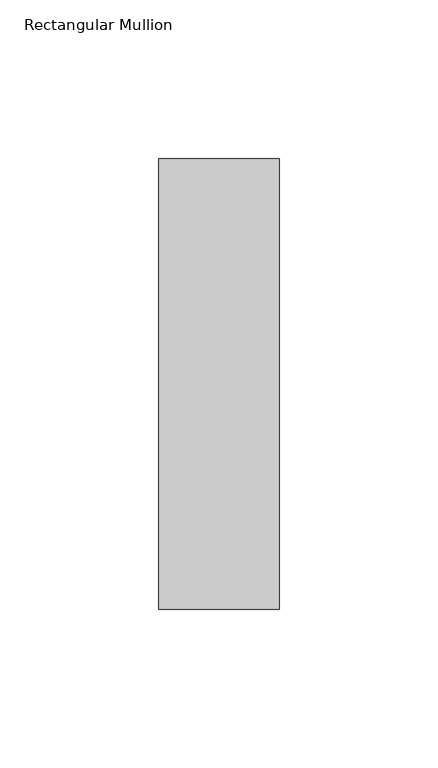
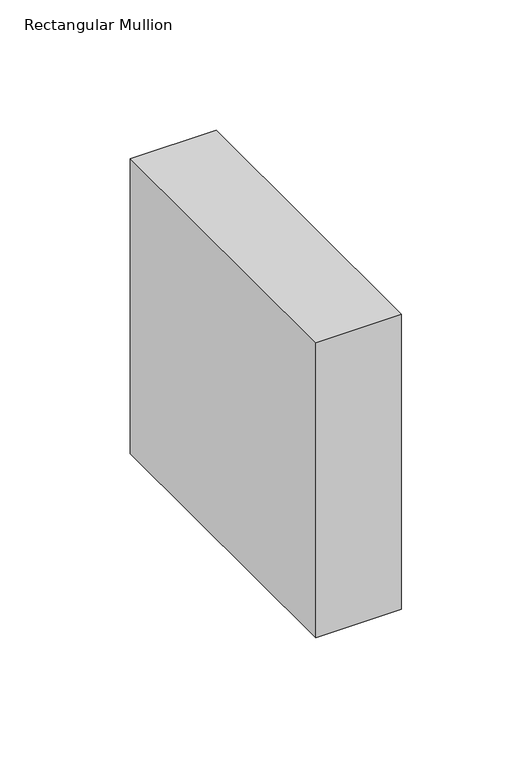
"""IFC4 building model written with IfcOpenShell, lengths in millimetres: member geometry, Rectangular Mullion : NLRS_21_CWM_hsb-regel 38x142_gen_rsf."""

import ifcopenshell
import ifcopenshell.guid

model = None  # the IFC model being written
_history = None  # IfcOwnerHistory: only IFC2X3 demands one
_inside = {}  # id of a spatial element -> (the spatial element, [elements in it])
_under = {}  # id of a project, library or spatial element -> (it, [spatial elements below it])
_declared = {}  # id of a project -> (the project, [libraries it declares])
_typed = {}  # id of a type object -> (the type object, [elements of that type])
_made_of = {}  # id of a material, layer set ... -> (it, [elements and type objects made of it])


def new_model(schema):
    """Start an empty IFC model of exactly this schema.

    Asked for "IFC4X3", IfcOpenShell would pick the latest addendum, in which some entities
    have other attributes; the version numbers below select the first issue.
    IFC2X3 requires an IfcOwnerHistory on every rooted entity: one is made here for all.
    """
    global model, _history
    if schema == "IFC4X3":
        model = ifcopenshell.file(schema_version=(4, 3, 0, 0))
    else:
        model = ifcopenshell.file(schema=schema)
    _inside.clear()
    _under.clear()
    _declared.clear()
    _typed.clear()
    _made_of.clear()
    _history = None
    if model.schema == "IFC2X3":
        org = make("IfcOrganization", Name="unknown")
        user = make(
            "IfcPersonAndOrganization",
            ThePerson=make("IfcPerson", FamilyName="unknown"),
            TheOrganization=org,
        )
        app = make(
            "IfcApplication",
            ApplicationDeveloper=org,
            Version="unknown",
            ApplicationFullName="unknown",
            ApplicationIdentifier="unknown",
        )
        _history = make(
            "IfcOwnerHistory",
            OwningUser=user,
            OwningApplication=app,
            ChangeAction="ADDED",
            CreationDate=0,
        )
    return model


def make(cls, **values):
    """One entity of the class cls with the attributes given. An attribute that is None is left unset."""
    return model.create_entity(
        cls, **{name: value for name, value in values.items() if value is not None}
    )


def rooted(cls, **values):
    """An entity with a GlobalId (a new one), such as an element, a storey or a relation."""
    return make(cls, GlobalId=ifcopenshell.guid.new(), OwnerHistory=_history, **values)


def si_unit(unit_type, name, prefix=None):
    """IfcSIUnit, for example si_unit("LENGTHUNIT", "METRE", prefix="MILLI")."""
    return make("IfcSIUnit", UnitType=unit_type, Prefix=prefix, Name=name)


def assignment(units):
    """IfcUnitAssignment: the units of a project."""
    return None if units is None else make("IfcUnitAssignment", Units=units)


def point(xyz):
    """IfcCartesianPoint."""
    return None if xyz is None else make("IfcCartesianPoint", Coordinates=xyz)


def direction(xyz):
    """IfcDirection."""
    return None if xyz is None else make("IfcDirection", DirectionRatios=xyz)


def frame(location, z_axis=None, x_axis=None):
    """IfcAxis2Placement3D, a coordinate frame: its origin and axes. An axis left out is left unset."""
    return make(
        "IfcAxis2Placement3D",
        Location=point(location),
        Axis=direction(z_axis),
        RefDirection=direction(x_axis),
    )


def origin():
    """The frame at (0, 0, 0) with its axes left unset."""
    return frame((0.0, 0.0, 0.0))


def place(relative_to, where):
    """IfcLocalPlacement: puts the frame where relative to a parent placement (None: the world)."""
    return make(
        "IfcLocalPlacement", PlacementRelTo=relative_to, RelativePlacement=where
    )


def context(
    kind, dimensions, precision=None, world=None, true_north=None, identifier=None
):
    """IfcGeometricRepresentationContext, for example the 3D "Model" context."""
    return make(
        "IfcGeometricRepresentationContext",
        ContextIdentifier=identifier,
        ContextType=kind,
        CoordinateSpaceDimension=dimensions,
        Precision=precision,
        WorldCoordinateSystem=world,
        TrueNorth=true_north,
    )


def project(units=None, contexts=None):
    """IfcProject with its units and contexts."""
    return rooted(
        "IfcProject",
        Name="project",
        RepresentationContexts=contexts,
        UnitsInContext=assignment(units),
    )


def spatial(cls, under=None, at=None, **own):
    """A site, building, storey or space (cls), placed at a placement, below another one or the project."""
    s = rooted(cls, ObjectPlacement=at, **own)
    if under is not None:
        _under.setdefault(under.id(), (under, []))[1].append(s)
    return s


def polyline(points):
    """IfcPolyline through the points."""
    return make("IfcPolyline", Points=[point(p) for p in points])


def outline(outer, holes=None, kind="AREA"):
    """IfcArbitraryClosedProfileDef: a profile drawn as a closed curve; with holes, ...WithVoids."""
    if holes is None:
        return make("IfcArbitraryClosedProfileDef", ProfileType=kind, OuterCurve=outer)
    return make(
        "IfcArbitraryProfileDefWithVoids",
        ProfileType=kind,
        OuterCurve=outer,
        InnerCurves=holes,
    )


def extrude(swept, where, along, depth):
    """IfcExtrudedAreaSolid: the profile swept, set in the frame where, extruded along a direction by depth."""
    return make(
        "IfcExtrudedAreaSolid",
        SweptArea=swept,
        Position=where,
        ExtrudedDirection=direction(along),
        Depth=depth,
    )


def shape(context_of_items, identifier, shape_type, items):
    """IfcShapeRepresentation: the items that make up one representation, for example the "Body"."""
    return make(
        "IfcShapeRepresentation",
        ContextOfItems=context_of_items,
        RepresentationIdentifier=identifier,
        RepresentationType=shape_type,
        Items=items,
    )


def source(mapping_origin, context_of_items, identifier, shape_type, items):
    """IfcRepresentationMap: a shape defined once, which mapped items show again and again."""
    return make(
        "IfcRepresentationMap",
        MappingOrigin=mapping_origin,
        MappedRepresentation=shape(context_of_items, identifier, shape_type, items),
    )


def transform(
    local_origin,
    x_axis=None,
    y_axis=None,
    z_axis=None,
    scale=None,
    scale2=None,
    scale3=None,
    uniform=True,
):
    """IfcCartesianTransformationOperator3D, or its non-uniform kind. x_axis, y_axis, z_axis: its Axis1, 2, 3."""
    if uniform:
        return make(
            "IfcCartesianTransformationOperator3D",
            Axis1=direction(x_axis),
            Axis2=direction(y_axis),
            LocalOrigin=point(local_origin),
            Scale=scale,
            Axis3=direction(z_axis),
        )
    return make(
        "IfcCartesianTransformationOperator3DnonUniform",
        Axis1=direction(x_axis),
        Axis2=direction(y_axis),
        LocalOrigin=point(local_origin),
        Scale=scale,
        Axis3=direction(z_axis),
        Scale2=scale2,
        Scale3=scale3,
    )


def mapped(mapping_source, mapping_target):
    """IfcMappedItem: shows the shape of a source again, moved by a transform."""
    return make(
        "IfcMappedItem", MappingSource=mapping_source, MappingTarget=mapping_target
    )


def made_of(thing, what):
    """Note that an element or type object is made of a material, layer set ...; save() writes the relation."""
    if what is not None:
        _made_of.setdefault(what.id(), (what, []))[1].append(thing)
    return thing


def element(
    cls,
    number,
    at=None,
    inside=None,
    cuts=None,
    type_object=None,
    material=None,
    context=None,
    identifier="Body",
    shape_type=None,
    held_by="IfcProductDefinitionShape",
    body=None,
    shapes=None,
    **own,
):
    """One element of the class cls, such as IfcWall. Its Tag is "e" and its number.

    at: its placement. inside: the storey or other place that contains it. cuts: it is an
    opening in that element (IfcRelVoidsElement). A single representation is given by context,
    identifier, shape_type and body (its items); several are given by shapes. held_by: the class
    of the entity that holds the representations. save() writes the other relations.
    """
    e = rooted(cls, Tag="e%d" % number, ObjectPlacement=at, **own)
    if body is not None:
        shapes = [shape(context, identifier, shape_type, body)]
    if shapes is not None:
        e.Representation = make(held_by, Representations=shapes)
    if inside is not None:
        _inside.setdefault(inside.id(), (inside, []))[1].append(e)
    if cuts is not None:
        rooted(
            "IfcRelVoidsElement", RelatingBuildingElement=cuts, RelatedOpeningElement=e
        )
    if type_object is not None:
        _typed.setdefault(type_object.id(), (type_object, []))[1].append(e)
    return made_of(e, material)


def aggregate(whole, parts):
    """IfcRelAggregates: a whole, such as a stair, and the parts it consists of."""
    return rooted("IfcRelAggregates", RelatingObject=whole, RelatedObjects=parts)


def save(model, path):
    """Write the relations noted so far, then the file.

    IfcRelAggregates (storeys below a building ...), IfcRelContainedInSpatialStructure (elements
    in a storey), IfcRelDefinesByType, IfcRelAssociatesMaterial and IfcRelDeclares: one each for
    every whole, place, type object, material and project.
    """
    for whole, parts in _under.values():
        aggregate(whole, parts)
    for where, things in _inside.values():
        rooted(
            "IfcRelContainedInSpatialStructure",
            RelatedElements=things,
            RelatingStructure=where,
        )
    for kind, things in _typed.values():
        rooted("IfcRelDefinesByType", RelatedObjects=things, RelatingType=kind)
    for what, things in _made_of.values():
        rooted("IfcRelAssociatesMaterial", RelatedObjects=things, RelatingMaterial=what)
    for by, libraries in _declared.values():
        rooted("IfcRelDeclares", RelatingContext=by, RelatedDefinitions=libraries)
    model.write(path)


def rectangular_mullion_d39b2c0b(model_context):
    return source(origin(), model_context, "Body", "SweptSolid", [
        extrude(outline(polyline([(-38.0, -71.0), (-38.0, 71.0), (0.0, 71.0), (0.0, -71.0), (-38.0, -71.0)])), frame((0.0, 0.0, -137.9999997), z_axis=(0.0, 0.0, 1.0), x_axis=(1.0, 0.0, 0.0)), (0.0, 0.0, 1.0), 137.9999997),
    ])


if __name__ == "__main__":
    model = new_model("IFC4")
    model_context = context("Model", 3, world=origin())
    ifc_project = project(units=[si_unit("LENGTHUNIT", "METRE", prefix="MILLI")], contexts=[model_context])
    site = spatial("IfcSite", under=ifc_project)
    building = spatial("IfcBuilding", under=site)
    placement = place(None, origin())
    rectangular_mullion_shape = rectangular_mullion_d39b2c0b(model_context)
    element("IfcMember", 1, ObjectType="Rectangular Mullion : NLRS_21_CWM_hsb-regel 38x142_gen_rsf", at=placement, inside=building, context=model_context, shape_type="MappedRepresentation", body=[
        mapped(rectangular_mullion_shape, transform((0.0, 0.0, 0.0), x_axis=(1.0, 0.0, 0.0), y_axis=(0.0, 1.0, 0.0), z_axis=(0.0, 0.0, 1.0))),
    ])
    save(model, "model.ifc")

# Revit data of these elements
# Type "Rectangular Mullion : NLRS_21_CWM_hsb-regel 38x142_gen_rsf"
#   Export Type to IFC As = "IfcWall"
#   Type IfcGUID = "07M7mRoiH1CR8m_RSKIwpF"
#   Assembly Code = "21.10"
#   built-in parameter 1007322 = 0.465879 (stored number, unit not read)
#   built-in parameter 1007321 = 0.062336 (stored number, unit not read)
#   built-in parameter 1007320 = 0.062336 (stored number, unit not read)
# Element 1 (IfcMember, "Rectangular Mullion : NLRS_21_CWM_hsb-regel 38x142_gen_rsf")
#   Materials on its faces: "NLRS_i2_hout naaldhout vuren_gen_rsf"
# Materials
#   "NLRS_i2_hout naaldhout vuren_gen_rsf": class "I - Hout", colour RGB 234 199 147, transparency 0, Keynote = "i2", Manufacturer = "Revit Standards Foundation", URL = "www.revitstandards.org", Description = "hout vuren", Cost = 0
